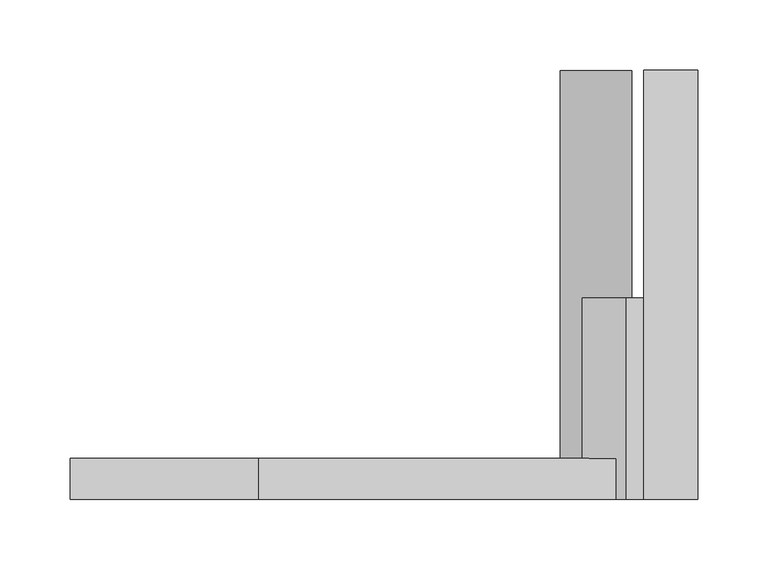
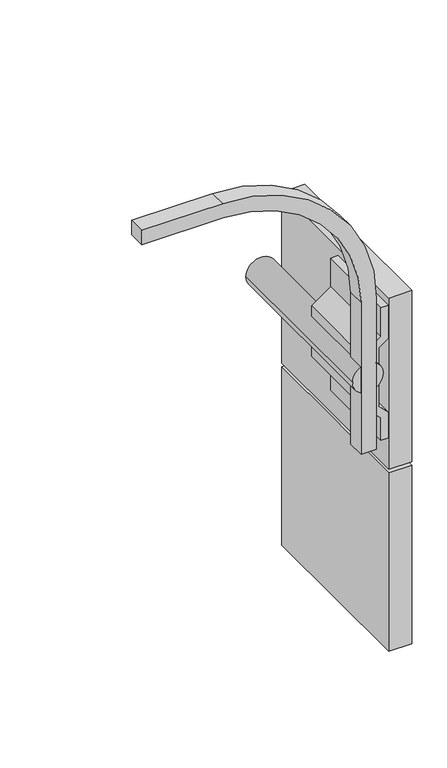
"""IFC4 building model written with IfcOpenShell, lengths in millimetres: proxy geometry, Generic Models 334:Generic Models 334:155354 : Generic Models 334:Generic Models 334:155354."""

from ifc_helpers import new_model, si_unit, point, frame, frame_2d, origin, place, context, project, spatial, polyline, circle_curve, trimmed, segment, composite_curve, outline, extrude, source, transform, mapped, element, save


def generic_models_ce0c9455(model_context):
    return source(origin(), model_context, "Body", "SweptSolid", [
        extrude(outline(polyline([(8206.5140422, -3919.5173293), (8206.5140422, -3614.7173293), (8244.6140422, -3614.7173293), (8244.6140422, -3919.5173293), (8206.5140422, -3919.5173293)])), frame((0.0, 0.0, 2591.8943036), z_axis=(0.0, 0.0, 1.0), x_axis=(1.0, 0.0, 0.0)), (0.0, 0.0, 1.0), 298.45),
        extrude(outline(polyline([(8206.5140422, -3919.5173293), (8206.5140422, -3614.7173293), (8244.6140422, -3614.7173293), (8244.6140422, -3919.5173293), (8206.5140422, -3919.5173293)])), frame((0.0, 0.0, 2274.3943036), z_axis=(0.0, 0.0, 1.0), x_axis=(1.0, 0.0, 0.0)), (0.0, 0.0, 1.0), 311.15),
        extrude(outline(composite_curve([segment(polyline([(2633.5611139, 8186.6937832), (2896.9926506, 8186.6937832)]), True, "CONTINUOUS"), segment(trimmed(circle_curve(frame_2d((2896.9926506, 7932.6937832)), 254.0), [point((2896.9926506, 8186.6937832))], [point((3150.9926506, 7932.6937832))], False, "CARTESIAN"), True, "CONTINUOUS"), segment(polyline([(3150.9926506, 7932.6937832), (3150.9926506, 7799.3437832), (3125.5926506, 7799.3437832), (3125.5926506, 7933.8945206)]), True, "CONTINUOUS"), segment(trimmed(circle_curve(frame_2d((2896.9926506, 7932.6937832)), 228.6031535), [point((3125.5926506, 7933.8945206))], [point((2898.1933881, 8161.2937832))], True, "CARTESIAN"), True, "CONTINUOUS"), segment(polyline([(2898.1933881, 8161.2937832), (2633.5611139, 8161.2937832), (2633.5611139, 8186.6937832)]), True, "CONTINUOUS")], self_intersect=False)), frame((0.0, -3919.5173293, 0.0), z_axis=(0.0, 1.0, 0.0), x_axis=(0.0, 0.0, 1.0)), (0.0, 0.0, 1.0), 28.9445755),
        extrude(outline(composite_curve([segment(trimmed(circle_curve(frame_2d((2763.2894905, 8172.5700497)), 25.4), [point((2763.2894905, 8197.9700497))], [point((2763.2894905, 8147.1700497))], False, "CARTESIAN"), True, "CONTINUOUS"), segment(trimmed(circle_curve(frame_2d((2763.2894905, 8172.5700497)), 25.4), [point((2763.2894905, 8147.1700497))], [point((2763.2894905, 8197.9700497))], False, "CARTESIAN"), True, "CONTINUOUS")], self_intersect=False)), frame((0.0, -3919.5173293, 0.0), z_axis=(0.0, 1.0, 0.0), x_axis=(0.0, 0.0, 1.0)), (0.0, 0.0, 1.0), 304.8),
        extrude(outline(polyline([(2809.6153085, 8190.5511433), (2820.7926506, 8206.5140422), (2877.9426506, 8206.5140422), (2877.9426506, 8193.8140422), (2827.4038522, 8193.8140422), (2805.5505899, 8162.6043493), (2717.4788762, 8162.6043493), (2686.2691833, 8193.8140422), (2647.0796955, 8193.8140422), (2647.0796955, 8206.5140422), (2691.5296955, 8206.5140422), (2707.4925944, 8190.5511433), (2809.6153085, 8190.5511433)])), frame((0.0, -3919.5173293, 0.0), z_axis=(0.0, 1.0, 0.0), x_axis=(0.0, 0.0, 1.0)), (0.0, 0.0, 1.0), 143.0193921),
    ])


if __name__ == "__main__":
    model = new_model("IFC4")
    model_context = context("Model", 3, world=origin())
    ifc_project = project(units=[si_unit("LENGTHUNIT", "METRE", prefix="MILLI")], contexts=[model_context])
    site = spatial("IfcSite", under=ifc_project)
    building = spatial("IfcBuilding", under=site)
    placement = place(None, origin())
    generic_models_shape = generic_models_ce0c9455(model_context)
    element("IfcBuildingElementProxy", 1, Name="Generic Models 334:Generic Models 334:155354 : Generic Models 334:Generic Models 334:155354", ObjectType="Generic Models 334:Generic Models 334:155354 : Generic Models 334:Generic Models 334:155354", at=placement, inside=building, context=model_context, shape_type="MappedRepresentation", body=[
        mapped(generic_models_shape, transform((0.0, 0.0, 0.0), x_axis=(1.0, 0.0, 0.0), y_axis=(0.0, 1.0, 0.0), z_axis=(0.0, 0.0, 1.0))),
    ])
    save(model, "model.ifc")

# Revit data of these elements
# Type "Generic Models 334:Generic Models 334:155354 : Generic Models 334:Generic Models 334:155354"
#   NameOverride = "Generic Models 334:Generic Models 334:155354"
#   ObjectTypeOverride = "Generic Models 334:Generic Models 334"
#   Reference = "Generic Models 334"
#   Category = "Generic Models"
#   Tag = "155354"
# Element 1 (IfcBuildingElementProxy, "Generic Models 334:Generic Models 334:155354 : Generic Models 334:Generic Models 334:155354")
#   Materials on its faces: "_GARAGE DOOR TRACK", "_SECTIONAL WOODEN GARAGE DOOR PER SCHEDULE 31400"
# Materials
#   "_GARAGE DOOR TRACK": class "Metal", colour RGB 199 199 199, transparency 0, Description = "Structural steel 50ksi", Cost = 0
#   "_SECTIONAL WOODEN GARAGE DOOR PER SCHEDULE 31400": class "Unassigned", colour RGB 177 130 114, transparency 0
